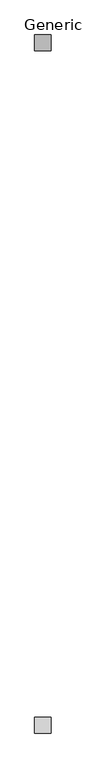
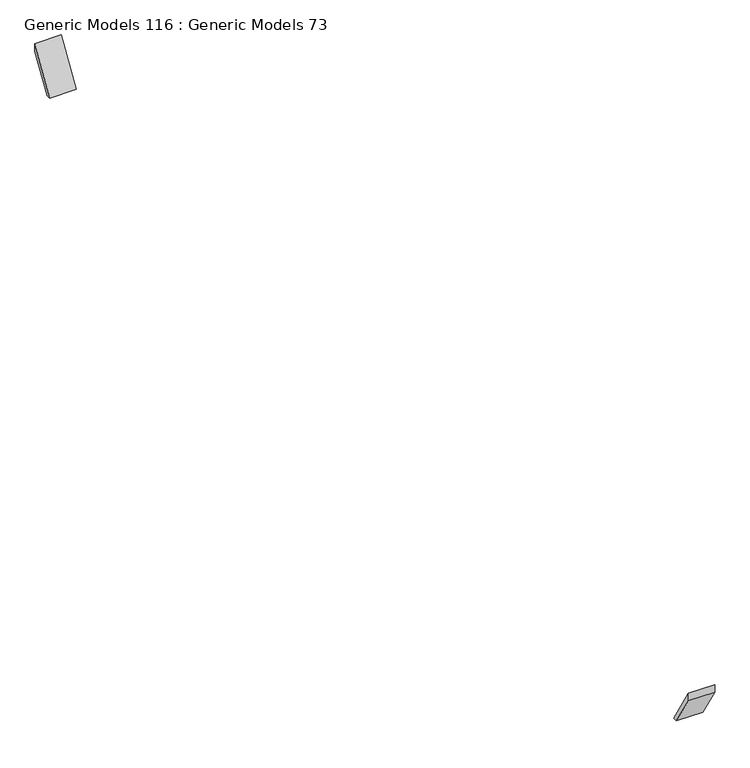
"""IFC4 building model written with IfcOpenShell, lengths in millimetres: proxy geometry, Generic Models 116 : Generic Models 73."""

from ifc_helpers import new_model, si_unit, frame, origin, place, context, project, spatial, polyline, outline, extrude, source, transform, mapped, element, save


def generic_models_116_generic_models_73_6fc075d3(model_context):
    return source(origin(), model_context, "Body", "SweptSolid", [
        extrude(outline(polyline([(30957.3619232, 266422.1875), (30940.0029838, 266422.1875), (30858.4781612, 266552.9810297), (30858.4781612, 266583.1406619), (30957.3619232, 266422.1875)])), frame((31924.6096032, 0.0, 0.0), z_axis=(1.0, 0.0, 0.0), x_axis=(0.0, 1.0, 0.0)), (0.0, 0.0, 1.0), 101.6),
        extrude(outline(polyline([(35106.7995322, 266422.1875), (35205.6832942, 266583.1406619), (35205.6832942, 266552.9810297), (35124.1584716, 266422.1875), (35106.7995322, 266422.1875)])), frame((31924.6096032, 0.0, 0.0), z_axis=(1.0, 0.0, 0.0), x_axis=(0.0, 1.0, 0.0)), (0.0, 0.0, 1.0), 101.6),
    ])


if __name__ == "__main__":
    model = new_model("IFC4")
    model_context = context("Model", 3, world=origin())
    ifc_project = project(units=[si_unit("LENGTHUNIT", "METRE", prefix="MILLI")], contexts=[model_context])
    site = spatial("IfcSite", under=ifc_project)
    building = spatial("IfcBuilding", under=site)
    placement = place(None, origin())
    generic_models_116_generic_models_73_shape = generic_models_116_generic_models_73_6fc075d3(model_context)
    element("IfcBuildingElementProxy", 1, Name="Generic Models 116 : Generic Models 73", ObjectType="Generic Models 116 : Generic Models 73", at=placement, inside=building, context=model_context, shape_type="MappedRepresentation", body=[
        mapped(generic_models_116_generic_models_73_shape, transform((0.0, 0.0, 0.0), x_axis=(1.0, 0.0, 0.0), y_axis=(0.0, 1.0, 0.0), z_axis=(0.0, 0.0, 1.0))),
    ])
    save(model, "model.ifc")

# Revit data of these elements
# Element 1 (IfcBuildingElementProxy, "Generic Models 116 : Generic Models 73")
#   Materials on its faces: "5/8\" x 4\"PLATE"
# Materials
#   "5/8\" x 4\"PLATE": class "Metal", colour RGB 199 199 199, transparency 0, Description = "Carbon steel", Cost = 0
